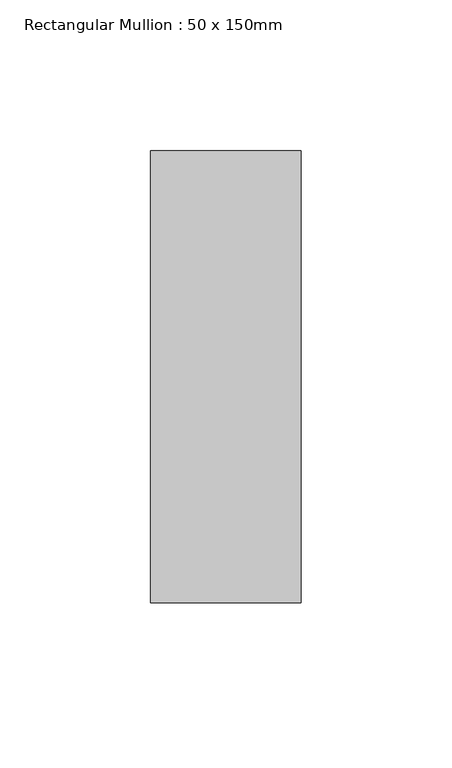
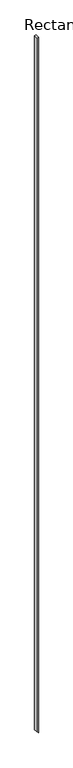
"""IFC4 building model written with IfcOpenShell, lengths in millimetres: member geometry, Rectangular Mullion : 50 x 150mm."""

from ifc_helpers import new_model, si_unit, frame, origin, place, context, project, spatial, polyline, outline, extrude, source, transform, mapped, element, save


def rectangular_mullion_50_x_150mm_b203450d(model_context):
    return source(origin(), model_context, "Body", "SweptSolid", [
        extrude(outline(polyline([(0.0, 0.0), (-16.6341861, -50.0), (-27709.4619673, -50.0), (-27756.5354594, 0.0), (0.0, 0.0)])), frame((0.0, -75.0, 0.0), z_axis=(0.0, 1.0, 0.0), x_axis=(0.0, 0.0, 1.0)), (0.0, 0.0, 1.0), 150.0),
    ])


if __name__ == "__main__":
    model = new_model("IFC4")
    model_context = context("Model", 3, world=origin())
    ifc_project = project(units=[si_unit("LENGTHUNIT", "METRE", prefix="MILLI")], contexts=[model_context])
    site = spatial("IfcSite", under=ifc_project)
    building = spatial("IfcBuilding", under=site)
    placement = place(None, origin())
    rectangular_mullion_50_x_150mm_shape = rectangular_mullion_50_x_150mm_b203450d(model_context)
    element("IfcMember", 1, ObjectType="Rectangular Mullion : 50 x 150mm", at=placement, inside=building, context=model_context, shape_type="MappedRepresentation", body=[
        mapped(rectangular_mullion_50_x_150mm_shape, transform((0.0, 0.0, 0.0), x_axis=(1.0, 0.0, 0.0), y_axis=(0.0, 1.0, 0.0), z_axis=(0.0, 0.0, 1.0))),
    ])
    save(model, "model.ifc")

# Revit data of these elements
# Type "Rectangular Mullion : 50 x 150mm"
#   built-in parameter 1007304 = 0.492126 (stored number, unit not read)
#   built-in parameter 1007301 = 0.082021 (stored number, unit not read)
#   built-in parameter 1007300 = 0.082021 (stored number, unit not read)
# Element 1 (IfcMember, "Rectangular Mullion : 50 x 150mm")
#   Materials on its faces: "Metal - Aluminium"
# Materials
#   "Metal - Aluminium": class "Metal", colour RGB 247 247 247, transparency 0
